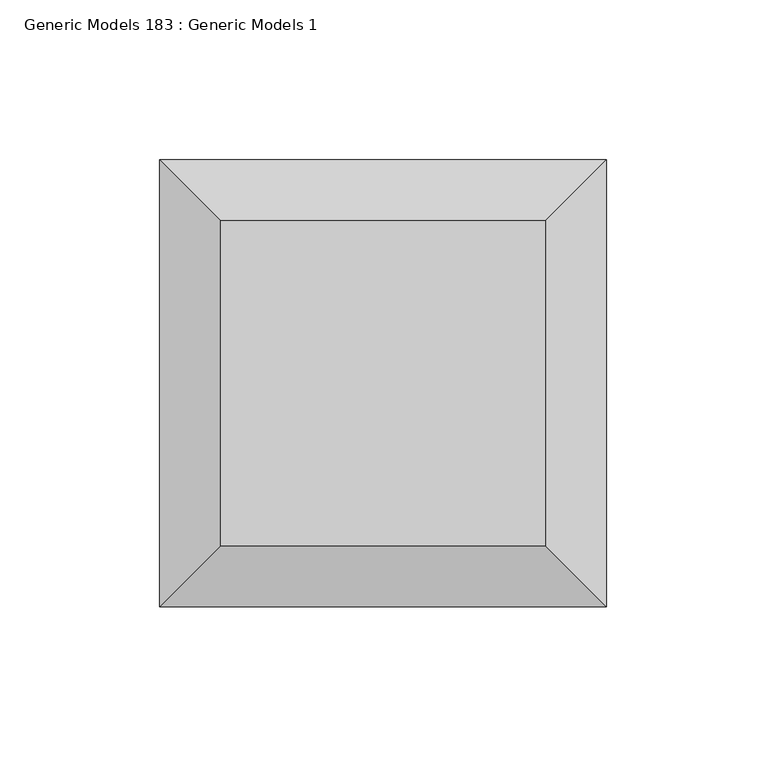
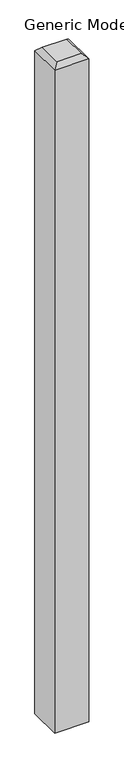
"""IFC4 building model written with IfcOpenShell, lengths in millimetres: proxy geometry, Generic Models 183 : Generic Models 1."""

import ifcopenshell
import ifcopenshell.guid

model = None  # the IFC model being written
_history = None  # IfcOwnerHistory: only IFC2X3 demands one
_inside = {}  # id of a spatial element -> (the spatial element, [elements in it])
_under = {}  # id of a project, library or spatial element -> (it, [spatial elements below it])
_declared = {}  # id of a project -> (the project, [libraries it declares])
_typed = {}  # id of a type object -> (the type object, [elements of that type])
_made_of = {}  # id of a material, layer set ... -> (it, [elements and type objects made of it])


def new_model(schema):
    """Start an empty IFC model of exactly this schema.

    Asked for "IFC4X3", IfcOpenShell would pick the latest addendum, in which some entities
    have other attributes; the version numbers below select the first issue.
    IFC2X3 requires an IfcOwnerHistory on every rooted entity: one is made here for all.
    """
    global model, _history
    if schema == "IFC4X3":
        model = ifcopenshell.file(schema_version=(4, 3, 0, 0))
    else:
        model = ifcopenshell.file(schema=schema)
    _inside.clear()
    _under.clear()
    _declared.clear()
    _typed.clear()
    _made_of.clear()
    _history = None
    if model.schema == "IFC2X3":
        org = make("IfcOrganization", Name="unknown")
        user = make(
            "IfcPersonAndOrganization",
            ThePerson=make("IfcPerson", FamilyName="unknown"),
            TheOrganization=org,
        )
        app = make(
            "IfcApplication",
            ApplicationDeveloper=org,
            Version="unknown",
            ApplicationFullName="unknown",
            ApplicationIdentifier="unknown",
        )
        _history = make(
            "IfcOwnerHistory",
            OwningUser=user,
            OwningApplication=app,
            ChangeAction="ADDED",
            CreationDate=0,
        )
    return model


def make(cls, **values):
    """One entity of the class cls with the attributes given. An attribute that is None is left unset."""
    return model.create_entity(
        cls, **{name: value for name, value in values.items() if value is not None}
    )


def rooted(cls, **values):
    """An entity with a GlobalId (a new one), such as an element, a storey or a relation."""
    return make(cls, GlobalId=ifcopenshell.guid.new(), OwnerHistory=_history, **values)


def si_unit(unit_type, name, prefix=None):
    """IfcSIUnit, for example si_unit("LENGTHUNIT", "METRE", prefix="MILLI")."""
    return make("IfcSIUnit", UnitType=unit_type, Prefix=prefix, Name=name)


def assignment(units):
    """IfcUnitAssignment: the units of a project."""
    return None if units is None else make("IfcUnitAssignment", Units=units)


def point(xyz):
    """IfcCartesianPoint."""
    return None if xyz is None else make("IfcCartesianPoint", Coordinates=xyz)


def direction(xyz):
    """IfcDirection."""
    return None if xyz is None else make("IfcDirection", DirectionRatios=xyz)


def frame(location, z_axis=None, x_axis=None):
    """IfcAxis2Placement3D, a coordinate frame: its origin and axes. An axis left out is left unset."""
    return make(
        "IfcAxis2Placement3D",
        Location=point(location),
        Axis=direction(z_axis),
        RefDirection=direction(x_axis),
    )


def origin():
    """The frame at (0, 0, 0) with its axes left unset."""
    return frame((0.0, 0.0, 0.0))


def place(relative_to, where):
    """IfcLocalPlacement: puts the frame where relative to a parent placement (None: the world)."""
    return make(
        "IfcLocalPlacement", PlacementRelTo=relative_to, RelativePlacement=where
    )


def context(
    kind, dimensions, precision=None, world=None, true_north=None, identifier=None
):
    """IfcGeometricRepresentationContext, for example the 3D "Model" context."""
    return make(
        "IfcGeometricRepresentationContext",
        ContextIdentifier=identifier,
        ContextType=kind,
        CoordinateSpaceDimension=dimensions,
        Precision=precision,
        WorldCoordinateSystem=world,
        TrueNorth=true_north,
    )


def project(units=None, contexts=None):
    """IfcProject with its units and contexts."""
    return rooted(
        "IfcProject",
        Name="project",
        RepresentationContexts=contexts,
        UnitsInContext=assignment(units),
    )


def spatial(cls, under=None, at=None, **own):
    """A site, building, storey or space (cls), placed at a placement, below another one or the project."""
    s = rooted(cls, ObjectPlacement=at, **own)
    if under is not None:
        _under.setdefault(under.id(), (under, []))[1].append(s)
    return s


def faces_of(points, faces, orient=None, outer=None):
    """IfcFace entities. A face is a list of loops; a loop is a list of indices into points, from 0.

    orient and outer hold one flag for each loop. By default every Orientation is true, the
    first loop of a face is its IfcFaceOuterBound and the others are IfcFaceBound.
    """
    made = []
    for i, loops in enumerate(faces):
        bounds = []
        for j, loop in enumerate(loops):
            is_outer = j == 0 if outer is None else outer[i][j]
            bounds.append(
                make(
                    "IfcFaceOuterBound" if is_outer else "IfcFaceBound",
                    Bound=make("IfcPolyLoop", Polygon=[points[k] for k in loop]),
                    Orientation=True if orient is None else orient[i][j],
                )
            )
        made.append(make("IfcFace", Bounds=bounds))
    return made


def faceted_brep(points, faces, orient=None, outer=None, voids=None):
    """IfcFacetedBrep: a solid bounded by flat faces; with voids (closed shells), ...WithVoids."""
    shared = [point(p) for p in points]
    hull = make("IfcClosedShell", CfsFaces=faces_of(shared, faces, orient, outer))
    if voids is None:
        return make("IfcFacetedBrep", Outer=hull)
    return make(
        "IfcFacetedBrepWithVoids",
        Outer=hull,
        Voids=[
            make(cls, CfsFaces=faces_of(shared, fs, o, b)) for cls, fs, o, b in voids
        ],
    )


def shape(context_of_items, identifier, shape_type, items):
    """IfcShapeRepresentation: the items that make up one representation, for example the "Body"."""
    return make(
        "IfcShapeRepresentation",
        ContextOfItems=context_of_items,
        RepresentationIdentifier=identifier,
        RepresentationType=shape_type,
        Items=items,
    )


def source(mapping_origin, context_of_items, identifier, shape_type, items):
    """IfcRepresentationMap: a shape defined once, which mapped items show again and again."""
    return make(
        "IfcRepresentationMap",
        MappingOrigin=mapping_origin,
        MappedRepresentation=shape(context_of_items, identifier, shape_type, items),
    )


def transform(
    local_origin,
    x_axis=None,
    y_axis=None,
    z_axis=None,
    scale=None,
    scale2=None,
    scale3=None,
    uniform=True,
):
    """IfcCartesianTransformationOperator3D, or its non-uniform kind. x_axis, y_axis, z_axis: its Axis1, 2, 3."""
    if uniform:
        return make(
            "IfcCartesianTransformationOperator3D",
            Axis1=direction(x_axis),
            Axis2=direction(y_axis),
            LocalOrigin=point(local_origin),
            Scale=scale,
            Axis3=direction(z_axis),
        )
    return make(
        "IfcCartesianTransformationOperator3DnonUniform",
        Axis1=direction(x_axis),
        Axis2=direction(y_axis),
        LocalOrigin=point(local_origin),
        Scale=scale,
        Axis3=direction(z_axis),
        Scale2=scale2,
        Scale3=scale3,
    )


def mapped(mapping_source, mapping_target):
    """IfcMappedItem: shows the shape of a source again, moved by a transform."""
    return make(
        "IfcMappedItem", MappingSource=mapping_source, MappingTarget=mapping_target
    )


def made_of(thing, what):
    """Note that an element or type object is made of a material, layer set ...; save() writes the relation."""
    if what is not None:
        _made_of.setdefault(what.id(), (what, []))[1].append(thing)
    return thing


def element(
    cls,
    number,
    at=None,
    inside=None,
    cuts=None,
    type_object=None,
    material=None,
    context=None,
    identifier="Body",
    shape_type=None,
    held_by="IfcProductDefinitionShape",
    body=None,
    shapes=None,
    **own,
):
    """One element of the class cls, such as IfcWall. Its Tag is "e" and its number.

    at: its placement. inside: the storey or other place that contains it. cuts: it is an
    opening in that element (IfcRelVoidsElement). A single representation is given by context,
    identifier, shape_type and body (its items); several are given by shapes. held_by: the class
    of the entity that holds the representations. save() writes the other relations.
    """
    e = rooted(cls, Tag="e%d" % number, ObjectPlacement=at, **own)
    if body is not None:
        shapes = [shape(context, identifier, shape_type, body)]
    if shapes is not None:
        e.Representation = make(held_by, Representations=shapes)
    if inside is not None:
        _inside.setdefault(inside.id(), (inside, []))[1].append(e)
    if cuts is not None:
        rooted(
            "IfcRelVoidsElement", RelatingBuildingElement=cuts, RelatedOpeningElement=e
        )
    if type_object is not None:
        _typed.setdefault(type_object.id(), (type_object, []))[1].append(e)
    return made_of(e, material)


def aggregate(whole, parts):
    """IfcRelAggregates: a whole, such as a stair, and the parts it consists of."""
    return rooted("IfcRelAggregates", RelatingObject=whole, RelatedObjects=parts)


def save(model, path):
    """Write the relations noted so far, then the file.

    IfcRelAggregates (storeys below a building ...), IfcRelContainedInSpatialStructure (elements
    in a storey), IfcRelDefinesByType, IfcRelAssociatesMaterial and IfcRelDeclares: one each for
    every whole, place, type object, material and project.
    """
    for whole, parts in _under.values():
        aggregate(whole, parts)
    for where, things in _inside.values():
        rooted(
            "IfcRelContainedInSpatialStructure",
            RelatedElements=things,
            RelatingStructure=where,
        )
    for kind, things in _typed.values():
        rooted("IfcRelDefinesByType", RelatedObjects=things, RelatingType=kind)
    for what, things in _made_of.values():
        rooted("IfcRelAssociatesMaterial", RelatedObjects=things, RelatingMaterial=what)
    for by, libraries in _declared.values():
        rooted("IfcRelDeclares", RelatingContext=by, RelatedDefinitions=libraries)
    model.write(path)


def generic_models_183_generic_models_1_4255d89c(model_context):
    return source(origin(), model_context, "Body", "Brep", [
        faceted_brep([(54227.4125, 528.6375, -1066.8), (54087.7125, 528.6375, -1066.8), (54087.7125, 528.6375, 1809.75), (54227.4125, 528.6375, 1809.75), (54227.4125, 388.9375, -1066.8), (54227.4125, 388.9375, 1809.75), (54087.7125, 388.9375, 1809.75), (54087.7125, 388.9375, -1066.8), (54106.7625, 407.9875, 1828.8), (54208.3625, 407.9875, 1828.8), (54208.3625, 509.5875, 1828.8), (54106.7625, 509.5875, 1828.8)], [[[0, 1, 2, 3]], [[4, 5, 6, 7]], [[1, 0, 4, 7]], [[2, 1, 7, 6]], [[8, 9, 10, 11]], [[0, 3, 5, 4]], [[2, 6, 8, 11]], [[5, 3, 10, 9]], [[6, 5, 9, 8]], [[3, 2, 11, 10]]]),
    ])


if __name__ == "__main__":
    model = new_model("IFC4")
    model_context = context("Model", 3, world=origin())
    ifc_project = project(units=[si_unit("LENGTHUNIT", "METRE", prefix="MILLI")], contexts=[model_context])
    site = spatial("IfcSite", under=ifc_project)
    building = spatial("IfcBuilding", under=site)
    placement = place(None, origin())
    generic_models_183_generic_models_1_shape = generic_models_183_generic_models_1_4255d89c(model_context)
    element("IfcBuildingElementProxy", 1, Name="Generic Models 183 : Generic Models 1", ObjectType="Generic Models 183 : Generic Models 1", at=placement, inside=building, context=model_context, shape_type="MappedRepresentation", body=[
        mapped(generic_models_183_generic_models_1_shape, transform((0.0, 0.0, 0.0), x_axis=(1.0, 0.0, 0.0), y_axis=(0.0, 1.0, 0.0), z_axis=(0.0, 0.0, 1.0))),
    ])
    save(model, "model.ifc")

# Revit data of these elements
# Element 1 (IfcBuildingElementProxy, "Generic Models 183 : Generic Models 1")
#   Materials on its faces: "TREATED CEDAR 6X6 POST"
# Materials
#   "TREATED CEDAR 6X6 POST": class "Wood", colour RGB 234 198 147, transparency 0, Description = "Pinus Echinata", Cost = 0
